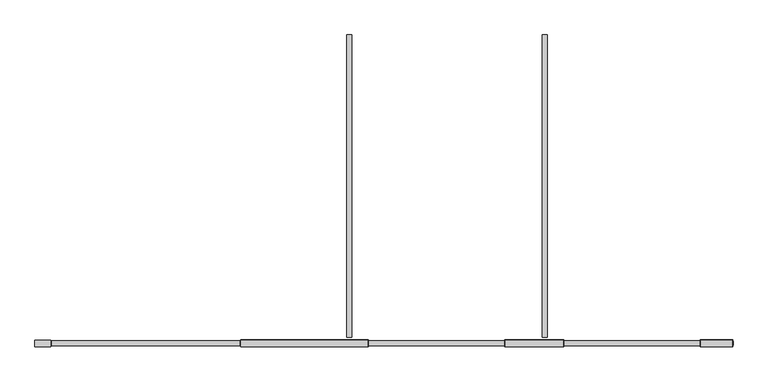
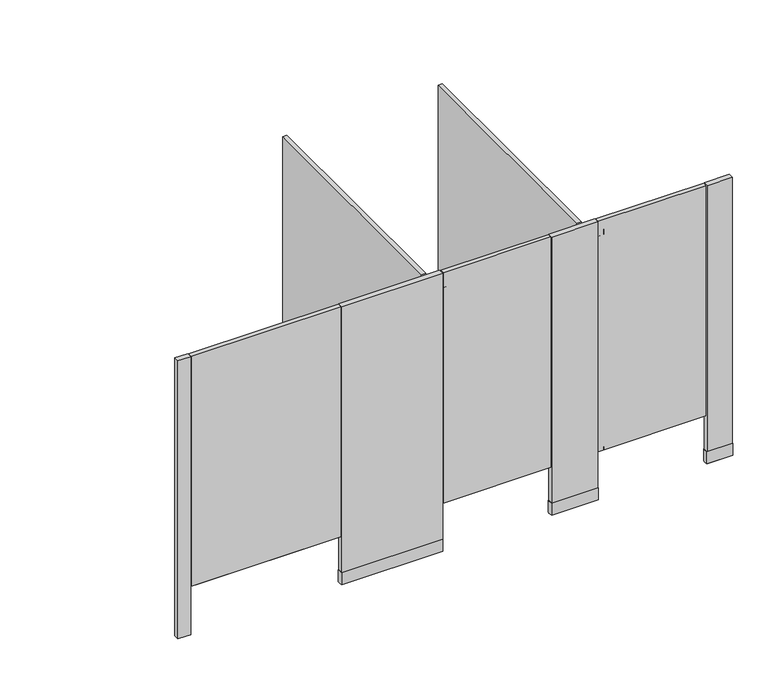
"""IFC4 building model written with IfcOpenShell, lengths in millimetres: proxy geometry, Partition-Floor_Braced-Bradley_Corp-St_Stl-ADA-N_Stalls : ADA (optional) + n Standard Stalls."""

from ifc_helpers import new_model, si_unit, point, frame, frame_2d, origin, origin_with_axes, place, context, project, spatial, polyline, circle_curve, trimmed, segment, composite_curve, outline, extrude, source, transform, mapped, element, save


def specialty_equipment_79de0914(model_context):
    return source(origin(), model_context, "Body", "SweptSolid", [
        extrude(outline(composite_curve([segment(polyline([(2474.9127547, -1487.4875), (2757.4891337, -1487.4875)]), True, "CONTINUOUS"), segment(trimmed(circle_curve(frame_2d((2701.700102, -1504.95)), 58.4581471), [point((2757.4891337, -1487.4875))], [point((2757.4891337, -1522.4125))], False, "CARTESIAN"), True, "CONTINUOUS"), segment(polyline([(2757.4891337, -1522.4125), (2474.9127547, -1522.4125)]), True, "CONTINUOUS"), segment(trimmed(circle_curve(frame_2d((2530.7017864, -1504.95)), 58.4581471), [point((2474.9127547, -1522.4125))], [point((2474.9127547, -1487.4875))], False, "CARTESIAN"), True, "CONTINUOUS")], self_intersect=False)), origin_with_axes(), (0.0, 0.0, 1.0), 76.2),
        extrude(outline(composite_curve([segment(polyline([(1204.9127547, -1487.4875), (1817.6891337, -1487.4875)]), True, "CONTINUOUS"), segment(trimmed(circle_curve(frame_2d((1761.900102, -1504.95)), 58.4581471), [point((1817.6891337, -1487.4875))], [point((1817.6891337, -1522.4125))], False, "CARTESIAN"), True, "CONTINUOUS"), segment(polyline([(1817.6891337, -1522.4125), (1204.9127547, -1522.4125)]), True, "CONTINUOUS"), segment(trimmed(circle_curve(frame_2d((1260.7017864, -1504.95)), 58.4581471), [point((1204.9127547, -1522.4125))], [point((1204.9127547, -1487.4875))], False, "CARTESIAN"), True, "CONTINUOUS")], self_intersect=False)), origin_with_axes(), (0.0, 0.0, 1.0), 76.2),
        extrude(outline(composite_curve([segment(polyline([(3414.7127547, -1487.4875), (3570.2891337, -1487.4875)]), True, "CONTINUOUS"), segment(trimmed(circle_curve(frame_2d((3514.500102, -1504.95)), 58.4581471), [point((3570.2891337, -1487.4875))], [point((3570.2891337, -1522.4125))], False, "CARTESIAN"), True, "CONTINUOUS"), segment(polyline([(3570.2891337, -1522.4125), (3414.7127547, -1522.4125)]), True, "CONTINUOUS"), segment(trimmed(circle_curve(frame_2d((3470.5017864, -1504.95)), 58.4581471), [point((3414.7127547, -1522.4125))], [point((3414.7127547, -1487.4875))], False, "CARTESIAN"), True, "CONTINUOUS")], self_intersect=False)), origin_with_axes(), (0.0, 0.0, 1.0), 76.2),
        extrude(outline(polyline([(1201.7250547, -1517.65), (296.8754547, -1517.65), (296.8754547, -1492.25), (1201.7250547, -1492.25), (1201.7250547, -1517.65)])), frame((0.0, 0.0, 304.8), z_axis=(0.0, 0.0, 1.0), x_axis=(1.0, 0.0, 0.0)), (0.0, 0.0, 1.0), 1473.2),
        extrude(outline(polyline([(3411.5250547, -1517.65), (2760.6754547, -1517.65), (2760.6754547, -1492.25), (3411.5250547, -1492.25), (3411.5250547, -1517.65)])), frame((0.0, 0.0, 304.8), z_axis=(0.0, 0.0, 1.0), x_axis=(1.0, 0.0, 0.0)), (0.0, 0.0, 1.0), 1473.2),
        extrude(outline(polyline([(2471.7250547, -1517.65), (1820.8754547, -1517.65), (1820.8754547, -1492.25), (2471.7250547, -1492.25), (2471.7250547, -1517.65)])), frame((0.0, 0.0, 304.8), z_axis=(0.0, 0.0, 1.0), x_axis=(1.0, 0.0, 0.0)), (0.0, 0.0, 1.0), 1473.2),
        extrude(outline(polyline([(304.8, 2471.7250547), (1778.0, 2471.7250547), (1778.0, 1820.8754547), (1714.5, 1820.8754547), (1714.5, 1852.6254547), (1682.75, 1852.6254547), (1682.75, 1820.8754547), (323.85, 1820.8754547), (323.85, 1852.6254547), (304.8, 1852.6254547), (304.8, 2471.7250547)])), frame((0.0, -1517.65, 0.0), z_axis=(0.0, 1.0, 0.0), x_axis=(0.0, 0.0, 1.0)), (0.0, 0.0, 1.0), 25.4),
        extrude(outline(polyline([(1778.0, 3411.5250547), (1778.0, 2760.6754547), (1714.5, 2760.6754547), (1714.5, 2792.4254547), (1682.75, 2792.4254547), (1682.75, 2760.6754547), (323.85, 2760.6754547), (323.85, 2792.4254547), (304.8, 2792.4254547), (304.8, 3411.5250547), (1778.0, 3411.5250547)])), frame((0.0, -1517.65, 0.0), z_axis=(0.0, 1.0, 0.0), x_axis=(0.0, 0.0, 1.0)), (0.0, 0.0, 1.0), 25.4),
        extrude(outline(polyline([(1778.0, 1201.7250547), (1778.0, 296.8754547), (1714.5, 296.8754547), (1714.5, 328.6254547), (1682.75, 328.6254547), (1682.75, 296.8754547), (323.85, 296.8754547), (323.85, 328.6254547), (304.8, 328.6254547), (304.8, 1201.7250547), (1778.0, 1201.7250547)])), frame((0.0, -1517.65, 0.0), z_axis=(0.0, 1.0, 0.0), x_axis=(0.0, 0.0, 1.0)), (0.0, 0.0, 1.0), 25.4),
        extrude(outline(polyline([(3416.3002547, -1489.075), (3568.7002547, -1489.075), (3568.7002547, -1520.825), (3416.3002547, -1520.825), (3416.3002547, -1489.075)])), origin_with_axes(), (0.0, 0.0, 1.0), 1778.0),
        extrude(outline(polyline([(2476.5002547, -1489.075), (2755.9002547, -1489.075), (2755.9002547, -1520.825), (2476.5002547, -1520.825), (2476.5002547, -1489.075)])), origin_with_axes(), (0.0, 0.0, 1.0), 1778.0),
        extrude(outline(polyline([(1206.5002547, -1489.075), (1816.1002547, -1489.075), (1816.1002547, -1520.825), (1206.5002547, -1520.825), (1206.5002547, -1489.075)])), origin_with_axes(), (0.0, 0.0, 1.0), 1778.0),
        extrude(outline(polyline([(215.9002547, -1489.075), (292.1002547, -1489.075), (292.1002547, -1520.825), (215.9002547, -1520.825), (215.9002547, -1489.075)])), origin_with_axes(), (0.0, 0.0, 1.0), 1778.0),
        extrude(outline(polyline([(2654.3002547, -1476.375), (2654.3002547, -22.225), (2679.7002547, -22.225), (2679.7002547, -1476.375), (2654.3002547, -1476.375)])), frame((0.0, 0.0, 304.8), z_axis=(0.0, 0.0, 1.0), x_axis=(1.0, 0.0, 0.0)), (0.0, 0.0, 1.0), 1473.2),
        extrude(outline(polyline([(1714.5002547, -1476.375), (1714.5002547, -22.225), (1739.9002547, -22.225), (1739.9002547, -1476.375), (1714.5002547, -1476.375)])), frame((0.0, 0.0, 304.8), z_axis=(0.0, 0.0, 1.0), x_axis=(1.0, 0.0, 0.0)), (0.0, 0.0, 1.0), 1473.2),
    ])


if __name__ == "__main__":
    model = new_model("IFC4")
    model_context = context("Model", 3, world=origin())
    ifc_project = project(units=[si_unit("LENGTHUNIT", "METRE", prefix="MILLI")], contexts=[model_context])
    site = spatial("IfcSite", under=ifc_project)
    building = spatial("IfcBuilding", under=site)
    placement = place(None, origin())
    specialty_equipment_shape = specialty_equipment_79de0914(model_context)
    element("IfcBuildingElementProxy", 1, Name="Partition-Floor_Braced-Bradley_Corp-St_Stl-ADA-N_Stalls : ADA (optional) + n Standard Stalls", ObjectType="Partition-Floor_Braced-Bradley_Corp-St_Stl-ADA-N_Stalls : ADA (optional) + n Standard Stalls", at=placement, inside=building, context=model_context, shape_type="MappedRepresentation", body=[
        mapped(specialty_equipment_shape, transform((0.0, 0.0, 0.0), x_axis=(1.0, 0.0, 0.0), y_axis=(0.0, 1.0, 0.0), z_axis=(0.0, 0.0, 1.0))),
    ])
    save(model, "model.ifc")

# Revit data of these elements
# Type "Partition-Floor_Braced-Bradley_Corp-St_Stl-ADA-N_Stalls : ADA (optional) + n Standard Stalls"
#   Keynote = "M10211313.01"
#   Warranty Information = "Warranted 15 years against rust out, 5 years on chrome hardware, lifetime of the partition on the stainless steel hardware."
#   Version = "1.3"
#   URL = "http://www.bradleycorp.com/"
#   Type Comments = "n/a"
#   Technical Data = "n/a"
#   Keynote = "M10211313.01"
#   OmniClass Title = "Toilet Compartment and Urinal Screens"
#   OmniClass Code = "23.15.11.15.11"
#   Modeling Code = "n/a"
#   Model = "Stainless Steel - Series 500 - Floor Braced"
#   Material Note = "Other Hardware Also Available - Please See www.bradleycorp.com"
#   Material = "Metal - Bradley Corp - Chrome"
#   MasterFormat Title = "Toilet Compartments"
#   MasterFormat Number = "10 21 13"
#   Manufacturer = "Bradley Corporation"
#   LEED Credit = ""
#   Industry Standards = "n/a"
#   Fire Rating = "n/a"
#   Description = "Restroom Partitions, Floor-Braced"
#   Copyright = "This Model Data is Property of Bradley Corporation"
#   Complies to NAFTA = "n/a"
#   Buy American Act = "To Be Determined"
#   Assembly Code = "C1010400"
#   ADA Compliant [instance default] = "Yes"
#   Width [instance default] = 11' - 5"
#   Top Hinge = 5' - 7"
#   Door Opening Standard [instance default] = 2' - 2"
#   Door Opening Angle [instance default] = 0.00°
#   MaskR [instance default] = 3' - 1"
#   Mask M [instance default] = 3' - 1"
#   Mask [instance default] = 5' - 1"
#   Shoe Height = 0' - 3"
#   RPn [instance default] = 0' - 1"
#   Pilaster Height = 5' - 10"
#   Latch to Edge = 0' - 2"
#   Latch Height = 3' - 1"
#   LPn [instance default] = 0' - 1"
#   Start STDA [instance default] = 0' - 0"
#   Start STD [instance default] = 5' - 5 1/2"
#   Start AMB [instance default] = 0' - 4 1/2"
#   Start STD2 [instance default] = 8' - 6 1/2"
#   Stall Width Standard [instance default] = 3' - 0"
#   Stall Depth [instance default] = 4' - 10 3/4"
#   Right Pilaster Width STD [instance default] = 0' - 3"
#   Pilaster Thickness = 0' - 1 1/4"
#   Percentage of Recycled Content = 0
#   Panel Thickness = 0' - 1"
#   Left Pilaster Width [instance default] = 0' - 4 1/2"
#   Height = 5' - 10"
#   Gap Side Wall Right [instance default] = 0' - 0"
#   Gap Side Wall Left [instance default] = 0' - 0"
#   Gap Pilaster Panel = 0' - 0 1/2"
#   Gap Back Wall [instance default] = 0' - 1"
#   End Right Pilaster = 0' - 0 1/2"
#   Door Width Standard [instance default] = 2' - 1.624"
#   Door Width ADA [instance default] = 2' - 11.624"
#   Door Thickness = 0' - 1"
#   Door Swing Angle [instance default] = 0.00°
#   Door Opening ADA [instance default] = 3' - 0"
#   Door Height = 4' - 10"
#   Door Handle Height = 3' - 1"
#   Door Gap = 0' - 0.188"
#   Depth [instance default] = 5' - 0"
#   CALC_Start STDs [instance default] = 5' - 5 1/2"
#   CALC_WidthA [instance default] = 3' - 1"
#   CALC_STDA Width [instance default] = 0' - 5"
#   CALC_STD2 Width [instance default] = 2' - 9"
#   CALC_RP [instance default] = 0' - 0"
#   CALC_Half Pilaster = 0' - 0 5/8"
#   CALC_Half Door Width = 0' - 11"
#   CALC_STD1 Width [instance default] = 2' - 9"
#   CALC_Left [instance default] = 0' - 4 1/2"
#   CALC_Half Panel = 0' - 0 1/2"
#   CALC_Angle [instance default] = 30.00°
#   CALC_AMB Width [instance default] = 4' - 9"
#   CALC_ADAngle [instance default] = 0.00°
#   CALC_ADADoorW [instance default] = 2' - 11.624"
#   CALC_ADADoorSwing [instance default] = 0.00°
#   CALC_ADADiff [instance default] = 2' - 0"
#   Bumper Height = 1' - 4"
#   Bottom Hinge = 1' - 0"
#   Bottom AFF = 1' - 0"
#   Brackets Top Height = 5' - 4"
#   Brackets Bottom Height = 1' - 6"
#   Right Pilaster Width AMB [instance default] = 0' - 3"
#   Stall Width ADA [instance default] = 5' - 0"
#   Outswing Door ADA [instance default] = yes
#   Instructions On-Off Visibility = yes
#   Outswing Door [instance default] = no
#   STDA [instance default] = no
#   STD2 [instance default] = yes
#   STD1 [instance default] = yes
#   RP STD2 [instance default] = yes
#   RP STD1 [instance default] = yes
#   RP AMB [instance default] = yes
#   Stalls Array [instance default] = 2
#   Right Panel [instance default] = yes
#   Stalls [instance default] = 3
#   Left Panel [instance default] = yes
#   Continuous Brackets [instance default] = yes
#   CALC_STD2Out [instance default] = no
#   CALC_STD1Out [instance default] = no
#   CALC_OutADA [instance default] = yes
#   CALC_NSTD2Out [instance default] = yes
#   CALC_NSTD1Out [instance default] = yes
#   CALC_NRP [instance default] = no
#   CALC_NOutADA [instance default] = no
#   CALC_NLF [instance default] = no
#   CALC_ADAOut [instance default] = yes
#   Brackets [instance default] = no
#   ADA Stall [instance default] = yes
#   Shoe Material = Metal - Bradley Corp - Stainless Steel Satin
#   Hardware Material = Metal - Bradley Corp - Chrome
#   Partition Material = Metal - Bradley Corp - Chrome
# Element 1 (IfcBuildingElementProxy, "Partition-Floor_Braced-Bradley_Corp-St_Stl-ADA-N_Stalls : ADA (optional) + n Standard Stalls")
#   Width = 11' - 2"
#   MaskR = 3' - 0 1/2"
#   Mask = 5' - 0 1/2"
#   RPn = 0' - 0"
#   LPn = 0' - 0"
#   Start STD = 5' - 4"
#   Start AMB = 0' - 4"
#   Start STD2 = 8' - 5"
#   Left Pilaster Width = 0' - 3"
#   Gap Side Wall Right = 0' - 1"
#   Gap Side Wall Left = 0' - 1"
#   CALC_Start STDs = 5' - 4"
#   CALC_STD2 Width = 2' - 6 1/2"
#   CALC_RP = -0' - 2 1/2"
#   CALC_Left = 0' - 4"
#   CALC_Angle = 0.00°
#   CALC_AMB Width = 4' - 8"
#   Outswing Door = yes
#   RP STD2 = no
#   Right Panel = no
#   Left Panel = no
#   CALC_STD2Out = yes
#   CALC_STD1Out = yes
#   CALC_NSTD2Out = no
#   CALC_NSTD1Out = no
#   CALC_NRP = yes
#   CALC_NLF = yes
#   Materials on its faces: "Metal - Bradley Corp - Chrome", "Metal - Bradley Corp - Stainless Steel Satin", "Plastic - Bradley Corp - Black"
# Materials
#   "Metal - Bradley Corp - Stainless Steel Satin": class "Metal", colour RGB 189 187 185, transparency 0
#   "Metal - Bradley Corp - Chrome": class "Metal", colour RGB 106 119 125, transparency 0, Cost = 0
#   "Plastic - Bradley Corp - Black": class "Plastic", colour RGB 5 5 5, transparency 0
